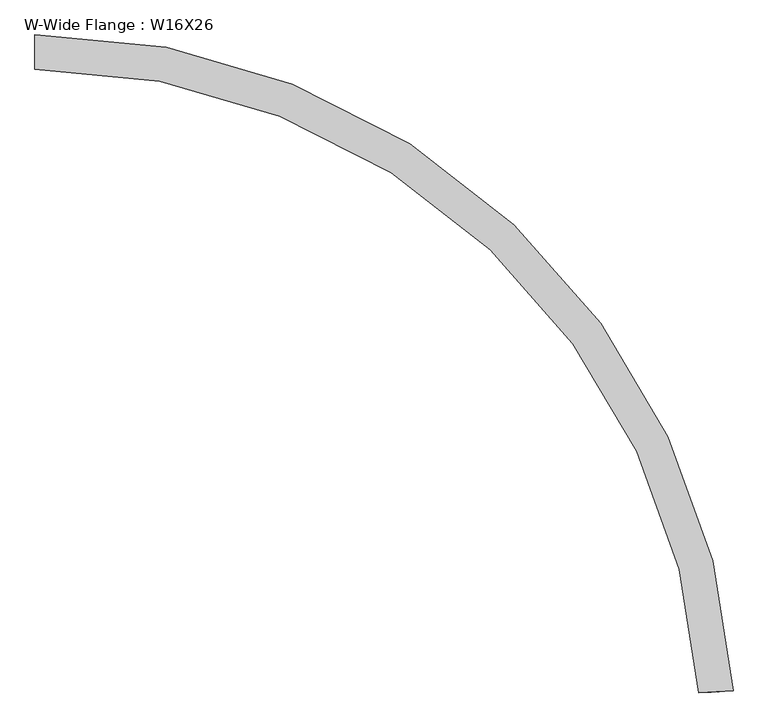
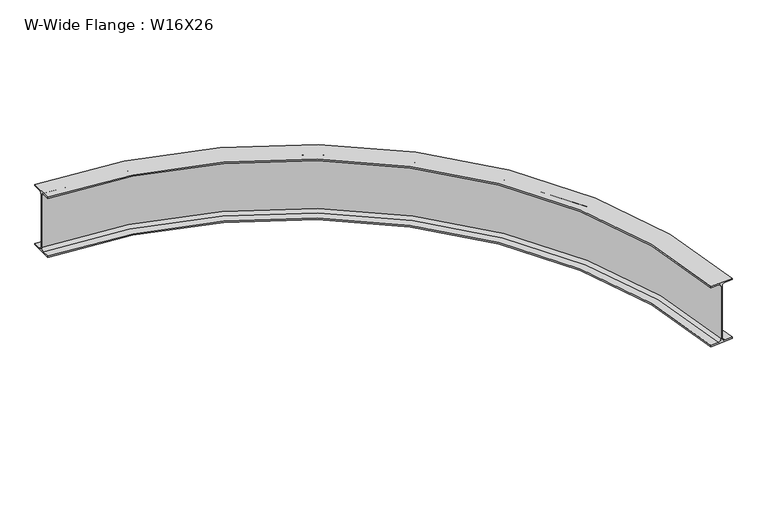
"""IFC4 building model written with IfcOpenShell, lengths in millimetres: beam geometry, W-Wide Flange : W16X26."""

from ifc_helpers import new_model, si_unit, point, frame, origin, place, context, project, spatial, polyline, circle_curve, ellipse_curve, trimmed, source, transform, mapped, element, save
from ifc_brep_helpers import plane_surface, cylinder_surface, revolved_surface, advanced_brep


def w_wide_flange_w16x26_9fbcf036(model_context):
    return source(origin(), model_context, "Body", "AdvancedBrep", [
        advanced_brep(
        [(2687.1196296, -2593.7096303, -190.5496094), (2687.1196296, -2593.7096303, -199.2808594), (2826.5456481, -2584.9646111, -199.2808594), (2826.5456481, -2584.9646111, -190.5496094), (2778.2218576, -2587.9955553, -190.5496094), (2760.001412, -2589.1383703, -172.2933594), (2760.001412, -2589.1383703, 172.2933594), (2778.2218576, -2587.9955553, 190.5496094), (2826.5456481, -2584.9646111, 190.5496094), (2826.5456481, -2584.9646111, 199.2808594), (2687.1196296, -2593.7096303, 199.2808594), (2687.1196296, -2593.7096303, 190.5496094), (2735.4434201, -2590.6786861, 190.5496094), (2753.6638657, -2589.5358711, 172.2933594), (2753.6638657, -2589.5358711, -172.2933594), (2735.4434201, -2590.6786861, -190.5496094), (0.0, -69.85, -190.5496094), (0.0, -21.43125, -190.5496094), (0.0, -3.175, -172.2933594), (0.0, -3.175, 172.2933594), (0.0, -21.43125, 190.5496094), (0.0, -69.85, 190.5496094), (0.0, -69.85, 199.2808594), (0.0, 69.85, 199.2808594), (0.0, 69.85, 190.5496094), (0.0, 21.43125, 190.5496094), (0.0, 3.175, 172.2933594), (0.0, 3.175, -172.2933594), (0.0, 21.43125, -190.5496094), (0.0, 69.85, -190.5496094), (0.0, 69.85, -199.2808594), (0.0, -69.85, -199.2808594)],
        [
            (0, 1),
            (1, 2),
            (2, 3),
            (3, 4),
            (4, 5, circle_curve(frame((2778.2218576, -2587.9955553, -172.2933594), z_axis=(-0.06259856251271431, 0.9980387868070768, 0.0), x_axis=(0.9980387868070768, 0.06259856251271431, 0.0)), 18.25625)),
            (5, 6),
            (6, 7, circle_curve(frame((2778.2218576, -2587.9955553, 172.2933594), z_axis=(-0.06259856251271431, 0.9980387868070768, 0.0), x_axis=(0.9980387868070768, 0.06259856251271431, 0.0)), 18.25625)),
            (7, 8),
            (8, 9),
            (9, 10),
            (10, 11),
            (11, 12),
            (12, 13, circle_curve(frame((2735.4434201, -2590.6786861, 172.2933594), z_axis=(-0.06259856251271431, 0.9980387868070768, 0.0), x_axis=(0.9980387868070768, 0.06259856251271431, 0.0)), 18.25625)),
            (13, 14),
            (14, 15, circle_curve(frame((2735.4434201, -2590.6786861, -172.2933594), z_axis=(-0.06259856251271431, 0.9980387868070768, 0.0), x_axis=(0.9980387868070768, 0.06259856251271431, 0.0)), 18.25625)),
            (15, 0),
            (16, 17),
            (17, 18, circle_curve(frame((0.0, -21.43125, -172.2933594), z_axis=(1.0, 0.0, 0.0), x_axis=(0.0, 1.0, 0.0)), 18.25625)),
            (18, 19),
            (19, 20, circle_curve(frame((0.0, -21.43125, 172.2933594), z_axis=(1.0, 0.0, 0.0), x_axis=(0.0, 1.0, 0.0)), 18.25625)),
            (20, 21),
            (21, 22),
            (22, 23),
            (23, 24),
            (24, 25),
            (25, 26, circle_curve(frame((0.0, 21.43125, 172.2933594), z_axis=(1.0, 0.0, 0.0), x_axis=(0.0, 1.0, 0.0)), 18.25625)),
            (26, 27),
            (27, 28, circle_curve(frame((0.0, 21.43125, -172.2933594), z_axis=(1.0, 0.0, 0.0), x_axis=(0.0, 1.0, 0.0)), 18.25625)),
            (28, 29),
            (29, 30),
            (30, 31),
            (31, 16),
            (15, 17, circle_curve(frame((0.0, -2762.25, -190.5496094), z_axis=(0.0, 0.0, 1.0), x_axis=(-1.0, 0.0, 0.0)), 2740.81875)),
            (16, 0, circle_curve(frame((0.0, -2762.25, -190.5496094), z_axis=(0.0, 0.0, -1.0), x_axis=(-1.0, 0.0, 0.0)), 2692.4)),
            (14, 18, circle_curve(frame((0.0, -2762.25, -172.2933594), z_axis=(0.0, 0.0, 1.0), x_axis=(-1.0, 0.0, 0.0)), 2759.075)),
            (13, 19, circle_curve(frame((0.0, -2762.25, 172.2933594), z_axis=(0.0, 0.0, 1.0), x_axis=(-1.0, 0.0, 0.0)), 2759.075)),
            (12, 20, circle_curve(frame((0.0, -2762.25, 190.5496094), z_axis=(0.0, 0.0, 1.0), x_axis=(-1.0, 0.0, 0.0)), 2740.81875)),
            (11, 21, circle_curve(frame((0.0, -2762.25, 190.5496094), z_axis=(0.0, 0.0, 1.0), x_axis=(-1.0, 0.0, 0.0)), 2692.4)),
            (10, 22, circle_curve(frame((0.0, -2762.25, 199.2808594), z_axis=(0.0, 0.0, 1.0), x_axis=(-1.0, 0.0, 0.0)), 2692.4)),
            (9, 23, circle_curve(frame((0.0, -2762.25, 199.2808594), z_axis=(0.0, 0.0, 1.0), x_axis=(-1.0, 0.0, 0.0)), 2832.1)),
            (8, 24, circle_curve(frame((0.0, -2762.25, 190.5496094), z_axis=(0.0, 0.0, 1.0), x_axis=(-1.0, 0.0, 0.0)), 2832.1)),
            (7, 25, circle_curve(frame((0.0, -2762.25, 190.5496094), z_axis=(0.0, 0.0, 1.0), x_axis=(-1.0, 0.0, 0.0)), 2783.68125)),
            (6, 26, circle_curve(frame((0.0, -2762.25, 172.2933594), z_axis=(0.0, 0.0, 1.0), x_axis=(-1.0, 0.0, 0.0)), 2765.425)),
            (5, 27, circle_curve(frame((0.0, -2762.25, -172.2933594), z_axis=(0.0, 0.0, 1.0), x_axis=(-1.0, 0.0, 0.0)), 2765.425)),
            (4, 28, circle_curve(frame((0.0, -2762.25, -190.5496094), z_axis=(0.0, 0.0, 1.0), x_axis=(-1.0, 0.0, 0.0)), 2783.68125)),
            (3, 29, circle_curve(frame((0.0, -2762.25, -190.5496094), z_axis=(0.0, 0.0, 1.0), x_axis=(-1.0, 0.0, 0.0)), 2832.1)),
            (2, 30, circle_curve(frame((0.0, -2762.25, -199.2808594), z_axis=(0.0, 0.0, 1.0), x_axis=(-1.0, 0.0, 0.0)), 2832.1)),
            (1, 31, circle_curve(frame((0.0, -2762.25, -199.2808594), z_axis=(0.0, 0.0, 1.0), x_axis=(-1.0, 0.0, 0.0)), 2692.4)),
        ],
        [
            plane_surface(frame((2756.8326389, -2589.3371207, 0.0), z_axis=(0.06259856251270805, -0.9980387868070772, 0.0), x_axis=(0.0, 0.0, 1.0))),
            plane_surface(frame((0.0, 0.0, 0.0), z_axis=(-1.0, 0.0, 0.0), x_axis=(0.0, 0.0, 1.0))),
            plane_surface(frame((0.0, -2762.25, -190.5496094), z_axis=(0.0, 0.0, 1.0), x_axis=(-1.0, 0.0, 0.0))),
            revolved_surface(trimmed(ellipse_curve(frame((-2740.81875, -2762.25, -172.2933594), z_axis=(0.0, -1.0, 0.0), x_axis=(-1.0, 0.0, 0.0)), 18.25625, 18.25625), [point((-2759.075, -2762.25, -172.2933594))], [point((-2740.81875, -2762.25, -190.5496094))], True, "CARTESIAN"), (0.0, -2762.25, 0.0), (0.0, 0.0, 1.0)),
            revolved_surface(polyline([(-2759.075, -2762.25, 172.2933594), (-2759.075, -2762.25, -172.2933594)]), (0.0, -2762.25, 0.0), (0.0, 0.0, 1.0)),
            revolved_surface(trimmed(ellipse_curve(frame((-2740.81875, -2762.25, 172.2933594), z_axis=(0.0, -1.0, 0.0), x_axis=(-1.0, 0.0, 0.0)), 18.25625, 18.25625), [point((-2740.81875, -2762.25, 190.5496094))], [point((-2759.075, -2762.25, 172.2933594))], True, "CARTESIAN"), (0.0, -2762.25, 0.0), (0.0, 0.0, 1.0)),
            plane_surface(frame((0.0, -2762.25, 190.5496094), z_axis=(0.0, 0.0, -1.0), x_axis=(-1.0, 0.0, 0.0))),
            revolved_surface(polyline([(-2692.4, -2762.25, 199.2808594), (-2692.4, -2762.25, 190.5496094)]), (0.0, -2762.25, 0.0), (0.0, 0.0, 1.0)),
            plane_surface(frame((0.0, -2762.25, 199.2808594), z_axis=(0.0, 0.0, 1.0), x_axis=(-1.0, 0.0, 0.0))),
            cylinder_surface(frame((0.0, -2762.25, 0.0), z_axis=(0.0, 0.0, 1.0), x_axis=(-1.0, 0.0, 0.0)), 2832.1),
            revolved_surface(trimmed(ellipse_curve(frame((-2783.68125, -2762.25, 172.2933594), z_axis=(0.0, -1.0, 0.0), x_axis=(-1.0, 0.0, 0.0)), 18.25625, 18.25625), [point((-2765.425, -2762.25, 172.2933594))], [point((-2783.68125, -2762.25, 190.5496094))], True, "CARTESIAN"), (0.0, -2762.25, 0.0), (0.0, 0.0, 1.0)),
            cylinder_surface(frame((0.0, -2762.25, 0.0), z_axis=(0.0, 0.0, 1.0), x_axis=(-1.0, 0.0, 0.0)), 2765.425),
            revolved_surface(trimmed(ellipse_curve(frame((-2783.68125, -2762.25, -172.2933594), z_axis=(0.0, -1.0, 0.0), x_axis=(-1.0, 0.0, 0.0)), 18.25625, 18.25625), [point((-2783.68125, -2762.25, -190.5496094))], [point((-2765.425, -2762.25, -172.2933594))], True, "CARTESIAN"), (0.0, -2762.25, 0.0), (0.0, 0.0, 1.0)),
            plane_surface(frame((0.0, -2762.25, -199.2808594), z_axis=(0.0, 0.0, -1.0), x_axis=(-1.0, 0.0, 0.0))),
            revolved_surface(polyline([(-2692.4, -2762.25, -190.5496094), (-2692.4, -2762.25, -199.2808594)]), (0.0, -2762.25, 0.0), (0.0, 0.0, 1.0)),
        ],
        [
            (0, [[1, 2, 3, 4, 5, 6, 7, 8, 9, 10, 11, 12, 13, 14, 15, 16]]),
            (1, [[17, 18, 19, 20, 21, 22, 23, 24, 25, 26, 27, 28, 29, 30, 31, 32]]),
            (2, [[33, -17, 34, -16]]),
            (3, [[35, -18, -33, -15]]),
            (4, [[36, -19, -35, -14]]),
            (5, [[37, -20, -36, -13]]),
            (6, [[38, -21, -37, -12]]),
            (7, [[39, -22, -38, -11]]),
            (8, [[40, -23, -39, -10]]),
            (9, [[41, -24, -40, -9]]),
            (6, [[42, -25, -41, -8]]),
            (10, [[43, -26, -42, -7]]),
            (11, [[44, -27, -43, -6]]),
            (12, [[45, -28, -44, -5]]),
            (2, [[46, -29, -45, -4]]),
            (9, [[47, -30, -46, -3]]),
            (13, [[48, -31, -47, -2]]),
            (14, [[-34, -32, -48, -1]]),
        ],
    ),
    ])


if __name__ == "__main__":
    model = new_model("IFC4")
    model_context = context("Model", 3, world=origin())
    ifc_project = project(units=[si_unit("LENGTHUNIT", "METRE", prefix="MILLI")], contexts=[model_context])
    site = spatial("IfcSite", under=ifc_project)
    building = spatial("IfcBuilding", under=site)
    placement = place(None, origin())
    w_wide_flange_w16x26_shape = w_wide_flange_w16x26_9fbcf036(model_context)
    element("IfcBeam", 1, ObjectType="W-Wide Flange : W16X26", at=placement, inside=building, context=model_context, shape_type="MappedRepresentation", body=[
        mapped(w_wide_flange_w16x26_shape, transform((0.0, 0.0, 0.0), x_axis=(1.0, 0.0, 0.0), y_axis=(0.0, 1.0, 0.0), z_axis=(0.0, 0.0, 1.0))),
    ])
    save(model, "model.ifc")

# Revit data of these elements
# Type "W-Wide Flange : W16X26"
#   Assembly Code = "B10"
#   W = 26
#   Start Extension Calculation [instance default] = 10' - 0"
#   Start Extension [instance default] = -0' - 0 1/2"
#   End Extension Calculation [instance default] = 10' - 0"
#   End Extension [instance default] = -0' - 0 1/2"
#   Length [instance default] = 5' - 0"
#   bf = 0' - 5 1/2"
#   d = 1' - 3 177/256"
#   k = 0' - 1 1/16"
#   k2 = 0' - 0 23/32"
#   tf = 0' - 0 11/32"
#   tw = 0' - 0 1/4"
#   A = 0.05 SF
#   Beam Material [instance default] = Metal - Steel - ASTM A992
# Element 1 (IfcBeam, "W-Wide Flange : W16X26")
#   Materials on its faces: "Metal - Steel - ASTM A992"
# Materials
#   "Metal - Steel - ASTM A992": class "Metal", colour RGB 128 0 0, transparency 0
